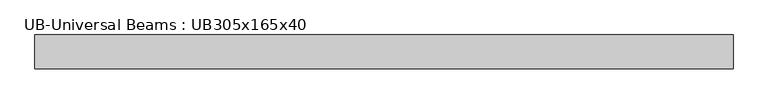
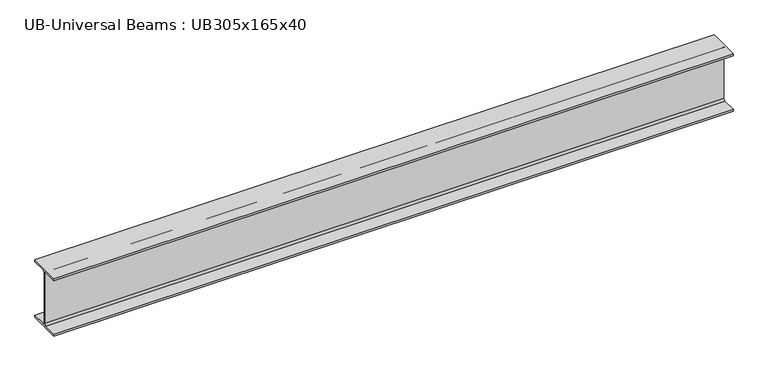
"""IFC4 building model written with IfcOpenShell, lengths in millimetres: member geometry, UB-Universal Beams : UB305x165x40."""

from ifc_helpers import new_model, si_unit, point, frame, frame_2d, origin, place, context, project, spatial, polyline, circle_curve, trimmed, segment, composite_curve, outline, extrude, source, transform, mapped, element, save


def ub_universal_beams_ub305x165x40_ae602ee7(model_context):
    return source(origin(), model_context, "Body", "SweptSolid", [
        extrude(outline(composite_curve([segment(polyline([(82.5, -141.5), (82.5, -151.7), (-82.5, -151.7), (-82.5, -141.5), (-11.9, -141.5)]), True, "CONTINUOUS"), segment(trimmed(circle_curve(frame_2d((-11.9, -132.6)), 8.9), [point((-11.9, -141.5))], [point((-3.0, -132.6))], True, "CARTESIAN"), True, "CONTINUOUS"), segment(polyline([(-3.0, -132.6), (-3.0, 132.6)]), True, "CONTINUOUS"), segment(trimmed(circle_curve(frame_2d((-11.9, 132.6)), 8.9), [point((-3.0, 132.6))], [point((-11.9, 141.5))], True, "CARTESIAN"), True, "CONTINUOUS"), segment(polyline([(-11.9, 141.5), (-82.5, 141.5), (-82.5, 151.7), (82.5, 151.7), (82.5, 141.5), (11.9, 141.5)]), True, "CONTINUOUS"), segment(trimmed(circle_curve(frame_2d((11.9, 132.6)), 8.9), [point((11.9, 141.5))], [point((3.0, 132.6))], True, "CARTESIAN"), True, "CONTINUOUS"), segment(polyline([(3.0, 132.6), (3.0, -132.6)]), True, "CONTINUOUS"), segment(trimmed(circle_curve(frame_2d((11.9, -132.6)), 8.9), [point((3.0, -132.6))], [point((11.9, -141.5))], True, "CARTESIAN"), True, "CONTINUOUS"), segment(polyline([(11.9, -141.5), (82.5, -141.5)]), True, "CONTINUOUS")], self_intersect=False)), frame((-1700.0, 0.0, 0.0), z_axis=(1.0, 0.0, 0.0), x_axis=(0.0, 1.0, 0.0)), (0.0, 0.0, 1.0), 3400.0),
    ])


if __name__ == "__main__":
    model = new_model("IFC4")
    model_context = context("Model", 3, world=origin())
    ifc_project = project(units=[si_unit("LENGTHUNIT", "METRE", prefix="MILLI")], contexts=[model_context])
    site = spatial("IfcSite", under=ifc_project)
    building = spatial("IfcBuilding", under=site)
    placement = place(None, origin())
    ub_universal_beams_ub305x165x40_shape = ub_universal_beams_ub305x165x40_ae602ee7(model_context)
    element("IfcMember", 1, ObjectType="UB-Universal Beams : UB305x165x40", at=placement, inside=building, context=model_context, shape_type="MappedRepresentation", body=[
        mapped(ub_universal_beams_ub305x165x40_shape, transform((0.0, 0.0, 0.0), x_axis=(1.0, 0.0, 0.0), y_axis=(0.0, 1.0, 0.0), z_axis=(0.0, 0.0, 1.0))),
    ])
    save(model, "model.ifc")

# Revit data of these elements
# Type "UB-Universal Beams : UB305x165x40"
#   Section Name Key = "UB305X165X40"
#   Width = 16.5 cm
#   Web Thickness = 0.6 cm
#   Web Fillet = 0.89 cm
#   Warping Constant = 164000.0 cm⁶
#   Torsional Moment of Inertia = 14.70 cm⁴
#   Section Area = 51.3 cm²
#   Plastic Modulus weak axis = 142.0 cm³
#   Plastic Modulus strong axis = 623.0 cm³
#   Nominal Weight = 40.2999 kgf/m
#   Moment of Inertia weak axis = 764.00 cm⁴
#   Moment of Inertia strong axis = 8503.00 cm⁴
#   Height = 30.34 cm
#   Flange Thickness = 1.02 cm
#   Elastic Modulus weak axis = 92.6 cm³
#   Elastic Modulus strong axis = 560.0 cm³
#   Centroid Vertical = 15.17 cm
#   Centroid Horizontal = 8.25 cm
#   Bolt Spacing = 9.0 cm
#   Length [instance default] = 1500 mm
#   Structural Material [instance default] = Metal - Steel 43-275
#   Type Comments = ""
#   Assembly Code = ""
# Element 1 (IfcMember, "UB-Universal Beams : UB305x165x40")
#   Materials on its faces: "Metal - Steel 43-275"
# Materials
#   "Metal - Steel 43-275": class "Metal", colour RGB 247 247 247, transparency 0, Cost = 0
